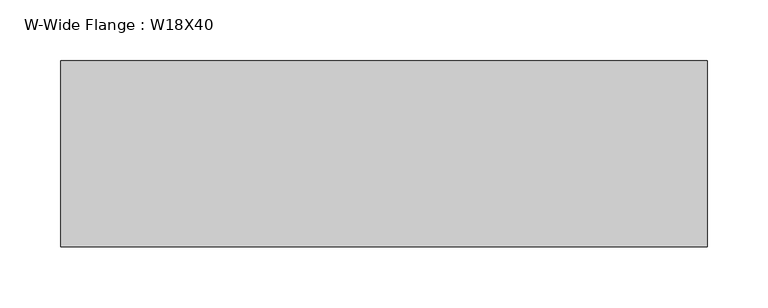
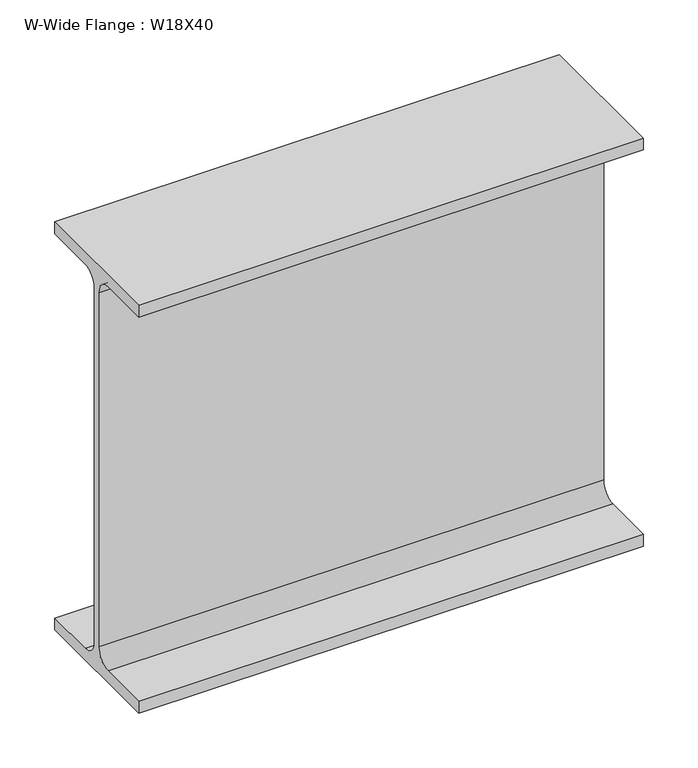
"""IFC4 building model written with IfcOpenShell, lengths in millimetres: beam geometry, W-Wide Flange : W18X40."""

from ifc_helpers import new_model, si_unit, point, frame, frame_2d, origin, place, context, project, spatial, polyline, circle_curve, trimmed, segment, composite_curve, outline, extrude, source, transform, mapped, element, save


def w_wide_flange_w18x40_6775d7a1(model_context):
    return source(origin(), model_context, "Body", "SweptSolid", [
        extrude(outline(composite_curve([segment(polyline([(76.454, -213.995), (76.454, -227.33), (-76.454, -227.33), (-76.454, -213.995), (-20.828, -213.995)]), True, "CONTINUOUS"), segment(trimmed(circle_curve(frame_2d((-20.828, -197.1675)), 16.8275), [point((-20.828, -213.995))], [point((-4.0005, -197.1675))], True, "CARTESIAN"), True, "CONTINUOUS"), segment(polyline([(-4.0005, -197.1675), (-4.0005, 197.1675)]), True, "CONTINUOUS"), segment(trimmed(circle_curve(frame_2d((-20.828, 197.1675)), 16.8275), [point((-4.0005, 197.1675))], [point((-20.828, 213.995))], True, "CARTESIAN"), True, "CONTINUOUS"), segment(polyline([(-20.828, 213.995), (-76.454, 213.995), (-76.454, 227.33), (76.454, 227.33), (76.454, 213.995), (20.828, 213.995)]), True, "CONTINUOUS"), segment(trimmed(circle_curve(frame_2d((20.828, 197.1675)), 16.8275), [point((20.828, 213.995))], [point((4.0005, 197.1675))], True, "CARTESIAN"), True, "CONTINUOUS"), segment(polyline([(4.0005, 197.1675), (4.0005, -197.1675)]), True, "CONTINUOUS"), segment(trimmed(circle_curve(frame_2d((20.828, -197.1675)), 16.8275), [point((4.0005, -197.1675))], [point((20.828, -213.995))], True, "CARTESIAN"), True, "CONTINUOUS"), segment(polyline([(20.828, -213.995), (76.454, -213.995)]), True, "CONTINUOUS")], self_intersect=False)), frame((-296.8625, 0.0, 0.0), z_axis=(1.0, 0.0, 0.0), x_axis=(0.0, 1.0, 0.0)), (0.0, 0.0, 1.0), 531.8125),
    ])


if __name__ == "__main__":
    model = new_model("IFC4")
    model_context = context("Model", 3, world=origin())
    ifc_project = project(units=[si_unit("LENGTHUNIT", "METRE", prefix="MILLI")], contexts=[model_context])
    site = spatial("IfcSite", under=ifc_project)
    building = spatial("IfcBuilding", under=site)
    placement = place(None, origin())
    w_wide_flange_w18x40_shape = w_wide_flange_w18x40_6775d7a1(model_context)
    element("IfcBeam", 1, ObjectType="W-Wide Flange : W18X40", at=placement, inside=building, context=model_context, shape_type="MappedRepresentation", body=[
        mapped(w_wide_flange_w18x40_shape, transform((0.0, 0.0, 0.0), x_axis=(1.0, 0.0, 0.0), y_axis=(0.0, 1.0, 0.0), z_axis=(0.0, 0.0, 1.0))),
    ])
    save(model, "model.ifc")

# Revit data of these elements
# Type "W-Wide Flange : W18X40"
#   Assembly Code = "B10"
#   W = 40
#   Length [instance default] = 5' - 0"
#   bf = 0' - 6.02"
#   d = 1' - 5.9"
#   k = 0' - 1 3/16"
#   k2 = 0' - 0.6625"
#   tf = 0' - 0.525"
#   tw = 0' - 0.315"
#   A = 0.0819444 SF
#   Structural Material [instance default] = Steel ASTM A992
# Element 1 (IfcBeam, "W-Wide Flange : W18X40")
#   Materials on its faces: "Steel ASTM A992"
# Materials
#   "Steel ASTM A992": class "Metal", colour RGB 199 199 199, transparency 0, Description = "Structural steel 50ksi", Cost = 0
